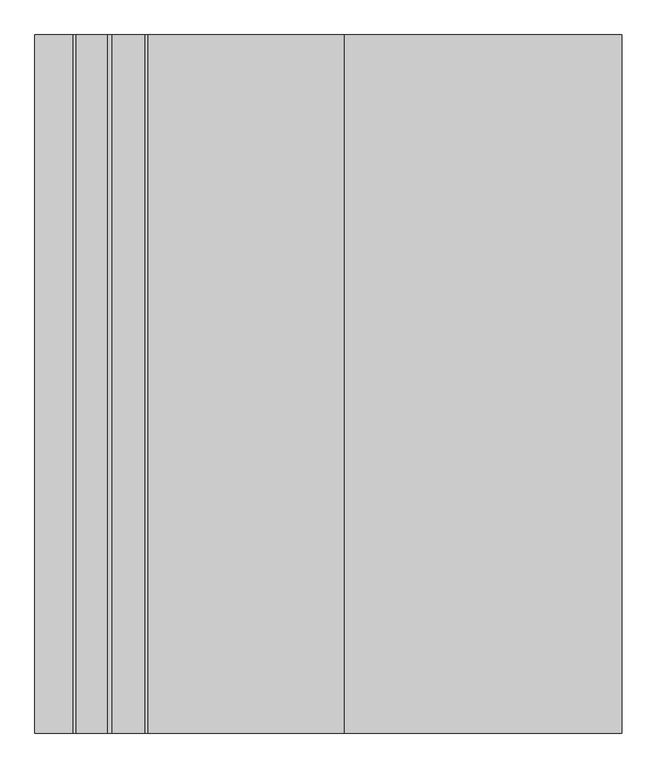
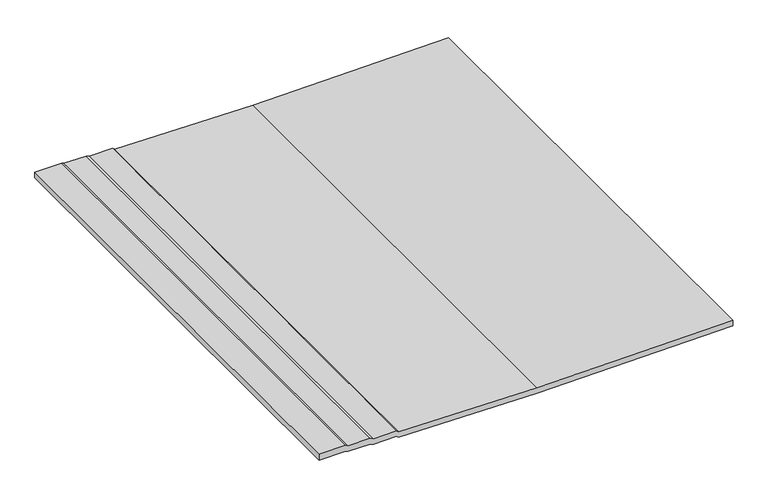
"""IFC4 building model written with IfcOpenShell, lengths in millimetres: proxy geometry, GRAVEL BALLAST004 14734 : GRAVEL BALLAST004 14734."""

from ifc_helpers import new_model, si_unit, frame, origin, place, context, project, spatial, polyline, outline, extrude, source, transform, mapped, element, save


def generic_models_1e64bb1d(model_context):
    return source(origin(), model_context, "Body", "SweptSolid", [
        extrude(outline(polyline([(40274.2359465, -2672.3662777), (40269.9546965, -2663.6558285), (40269.9546965, -2573.0689144), (40264.2272344, -2560.2242751), (40265.8726651, -2466.2725277), (40258.4625089, -2457.9990902), (40250.2437589, -1894.9286556), (40261.546875, -1099.1907959), (40286.2851563, -1099.1907959), (40274.9820403, -1894.9286556), (40283.2007903, -2457.9990902), (40290.6109465, -2466.2725277), (40288.9655158, -2560.2242751), (40294.6929777, -2573.0689144), (40294.6929777, -2663.6558285), (40298.9742278, -2672.3662777), (40298.9742278, -2781.8657894), (40274.2359465, -2781.8657894), (40274.2359465, -2672.3662777)])), frame((0.0, 1000.0, 0.0), z_axis=(0.0, 1.0, 0.0), x_axis=(0.0, 0.0, 1.0)), (0.0, 0.0, 1.0), 2000.0),
    ])


if __name__ == "__main__":
    model = new_model("IFC4")
    model_context = context("Model", 3, world=origin())
    ifc_project = project(units=[si_unit("LENGTHUNIT", "METRE", prefix="MILLI")], contexts=[model_context])
    site = spatial("IfcSite", under=ifc_project)
    building = spatial("IfcBuilding", under=site)
    placement = place(None, origin())
    generic_models_shape = generic_models_1e64bb1d(model_context)
    element("IfcBuildingElementProxy", 1, Name="GRAVEL BALLAST004 14734 : GRAVEL BALLAST004 14734", ObjectType="GRAVEL BALLAST004 14734 : GRAVEL BALLAST004 14734", at=placement, inside=building, context=model_context, shape_type="MappedRepresentation", body=[
        mapped(generic_models_shape, transform((0.0, 0.0, 0.0), x_axis=(1.0, 0.0, 0.0), y_axis=(0.0, 1.0, 0.0), z_axis=(0.0, 0.0, 1.0))),
    ])
    save(model, "model.ifc")

# Revit data of these elements
# Type "GRAVEL BALLAST004 14734 : GRAVEL BALLAST004 14734"
#   NameOverride = "GRAVEL BALLAST004"
# Element 1 (IfcBuildingElementProxy, "GRAVEL BALLAST004 14734 : GRAVEL BALLAST004 14734")
#   Materials on its faces: "GRAVEL BALLAST"
# Materials
#   "GRAVEL BALLAST": class "Unassigned", colour RGB 128 128 128, transparency 0, Cost = 0
